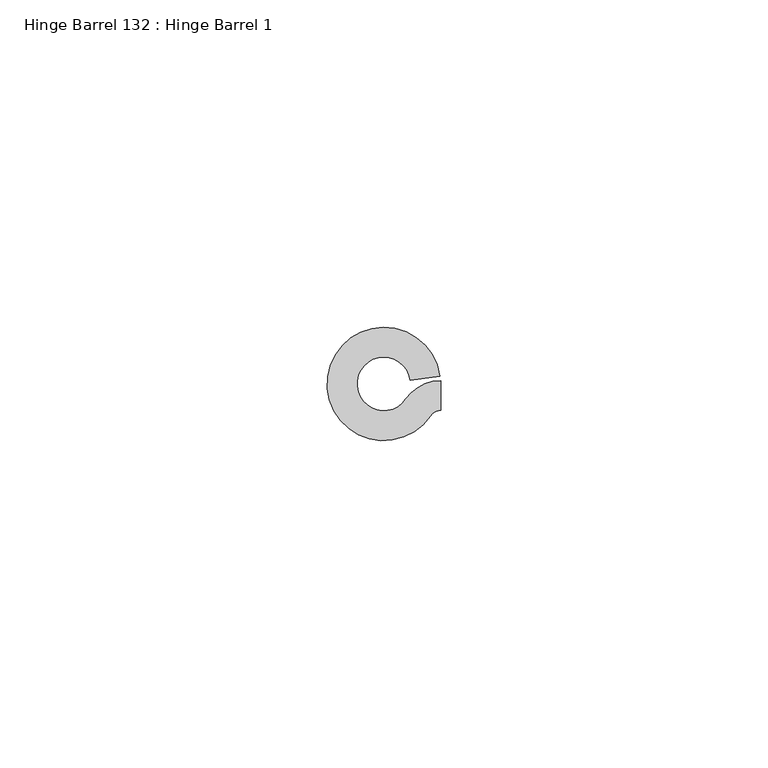
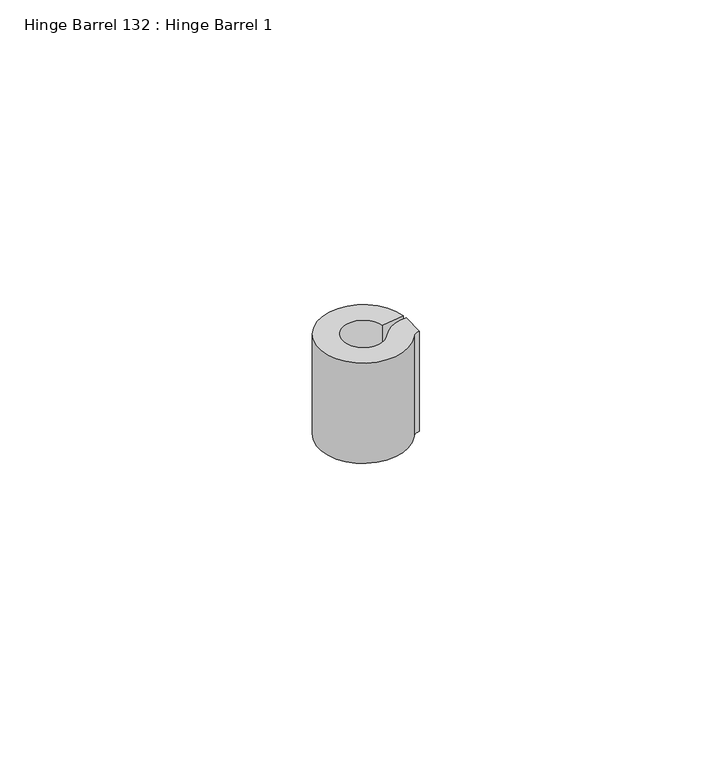
"""IFC4 building model written with IfcOpenShell, lengths in millimetres: proxy geometry, Hinge Barrel 132 : Hinge Barrel 1."""

from ifc_helpers import new_model, si_unit, point, frame, frame_2d, origin, place, context, project, spatial, polyline, circle_curve, trimmed, segment, composite_curve, outline, extrude, source, transform, mapped, element, save


def hinge_barrel_132_hinge_barrel_1_fe703ea2(model_context):
    return source(origin(), model_context, "Body", "SweptSolid", [
        extrude(outline(composite_curve([segment(trimmed(circle_curve(frame_2d((587327.8245257, -536316.2443067)), 6.4044851), [point((587322.5194669, -536312.6563017))], [point((587327.8245257, -536309.8398216))], False, "CARTESIAN"), True, "CONTINUOUS"), segment(polyline([(587327.8245257, -536309.8398216), (587327.8245257, -536314.4038841)]), True, "CONTINUOUS"), segment(trimmed(circle_curve(frame_2d((587327.8245257, -536316.2443067)), 1.8404226), [point((587327.8245257, -536314.4038841))], [point((587326.3000393, -536315.2132409))], True, "CARTESIAN"), True, "CONTINUOUS"), segment(trimmed(circle_curve(frame_2d((587319.1320739, -536310.3652841)), 8.6534625), [point((587326.3000393, -536315.2132409))], [point((587327.7022899, -536309.1678654))], False, "CARTESIAN"), True, "CONTINUOUS"), segment(polyline([(587327.7022899, -536309.1678654), (587323.1821338, -536309.7994153)]), True, "CONTINUOUS"), segment(trimmed(circle_curve(frame_2d((587319.1320739, -536310.3652841)), 4.0894), [point((587323.1821338, -536309.7994153))], [point((587322.5194669, -536312.6563017))], True, "CARTESIAN"), True, "CONTINUOUS")], self_intersect=False)), frame((0.0, 0.0, 438.15), z_axis=(0.0, 0.0, 1.0), x_axis=(1.0, 0.0, 0.0)), (0.0, 0.0, 1.0), 20.8359375),
    ])


if __name__ == "__main__":
    model = new_model("IFC4")
    model_context = context("Model", 3, world=origin())
    ifc_project = project(units=[si_unit("LENGTHUNIT", "METRE", prefix="MILLI")], contexts=[model_context])
    site = spatial("IfcSite", under=ifc_project)
    building = spatial("IfcBuilding", under=site)
    placement = place(None, origin())
    hinge_barrel_132_hinge_barrel_1_shape = hinge_barrel_132_hinge_barrel_1_fe703ea2(model_context)
    element("IfcBuildingElementProxy", 1, Name="Hinge Barrel 132 : Hinge Barrel 1", ObjectType="Hinge Barrel 132 : Hinge Barrel 1", at=placement, inside=building, context=model_context, shape_type="MappedRepresentation", body=[
        mapped(hinge_barrel_132_hinge_barrel_1_shape, transform((0.0, 0.0, 0.0), x_axis=(1.0, 0.0, 0.0), y_axis=(0.0, 1.0, 0.0), z_axis=(0.0, 0.0, 1.0))),
    ])
    save(model, "model.ifc")

# Revit data of these elements
# Element 1 (IfcBuildingElementProxy, "Hinge Barrel 132 : Hinge Barrel 1")
#   Materials on its faces: "6\"X6\" WELD-ON STL BUTT HINGE"
# Materials
#   "6\"X6\" WELD-ON STL BUTT HINGE": class "Metal", colour RGB 189 187 185, transparency 0, Description = "Carbon steel", Cost = 0
